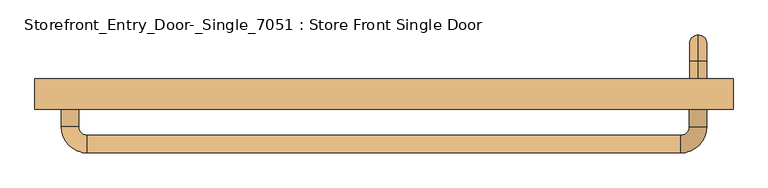
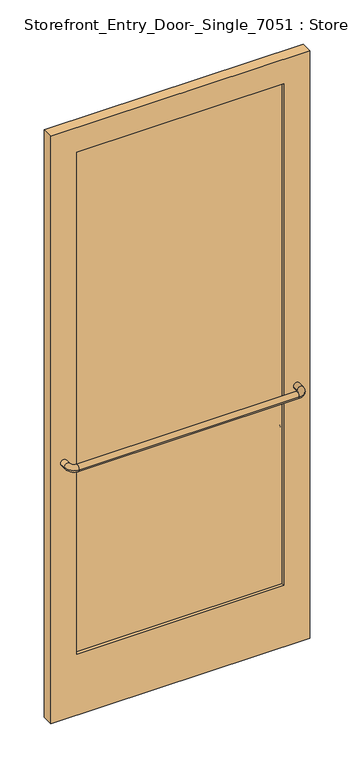
"""IFC4 building model written with IfcOpenShell, lengths in millimetres: door geometry, Storefront_Entry_Door-_Single_7051 : Store Front Single Door."""

from ifc_helpers import new_model, si_unit, point, frame, origin, place, context, project, spatial, polyline, circle_curve, ellipse_curve, trimmed, outline, extrude, source, transform, mapped, element, save
from ifc_brep_helpers import plane_surface, cylinder_surface, revolved_surface, advanced_brep


def storefront_entry_door_single_7051_store_front_single_door_f67f6f5c(model_context):
    return source(origin(), model_context, "Body", "SolidModel", [
        advanced_brep(
        [(457.2, 50.8, 1054.1), (457.2, 50.8, 1079.5), (457.2, 76.2, 1054.1), (457.2, 76.2, 1079.5), (457.2, 114.3, 1041.4), (457.2, 88.9, 1041.4), (457.2, 88.9, 863.6), (457.2, 114.3, 863.6), (457.2, 76.2, 825.5), (457.2, 76.2, 850.9), (457.2, 50.8, 850.9), (457.2, 50.8, 825.5)],
        [
            (0, 1, circle_curve(frame((457.2, 50.8, 1066.8), z_axis=(0.0, -1.0, 0.0), x_axis=(0.0, 0.0, 1.0)), 12.7)),
            (1, 0, circle_curve(frame((457.2, 50.8, 1066.8), z_axis=(0.0, -1.0, 0.0), x_axis=(0.0, 0.0, 1.0)), 12.7)),
            (0, 2),
            (2, 3, circle_curve(frame((457.2, 76.2, 1066.8), z_axis=(0.0, -1.0, 0.0), x_axis=(0.0, 0.0, 1.0)), 12.7)),
            (3, 1),
            (3, 2, circle_curve(frame((457.2, 76.2, 1066.8), z_axis=(0.0, -1.0, 0.0), x_axis=(0.0, 0.0, 1.0)), 12.7)),
            (4, 3, circle_curve(frame((457.2, 76.2, 1041.4), z_axis=(1.0, 0.0, 0.0), x_axis=(0.0, 0.0, 1.0)), 38.1)),
            (2, 5, circle_curve(frame((457.2, 76.2, 1041.4), z_axis=(-1.0, 0.0, 0.0), x_axis=(0.0, 0.0, 1.0)), 12.7)),
            (5, 4, circle_curve(frame((457.2, 101.6, 1041.4), z_axis=(0.0, 0.0, 1.0), x_axis=(0.0, 1.0, 0.0)), 12.7)),
            (4, 5, circle_curve(frame((457.2, 101.6, 1041.4), z_axis=(0.0, 0.0, 1.0), x_axis=(0.0, 1.0, 0.0)), 12.7)),
            (5, 6),
            (6, 7, circle_curve(frame((457.2, 101.6, 863.6), z_axis=(0.0, 0.0, 1.0), x_axis=(0.0, 1.0, 0.0)), 12.7)),
            (7, 4),
            (7, 6, circle_curve(frame((457.2, 101.6, 863.6), z_axis=(0.0, 0.0, 1.0), x_axis=(0.0, 1.0, 0.0)), 12.7)),
            (8, 7, circle_curve(frame((457.2, 76.2, 863.6), z_axis=(1.0, 0.0, 0.0), x_axis=(0.0, 1.0, 0.0)), 38.1)),
            (6, 9, circle_curve(frame((457.2, 76.2, 863.6), z_axis=(-1.0, 0.0, 0.0), x_axis=(0.0, 1.0, 0.0)), 12.7)),
            (9, 8, circle_curve(frame((457.2, 76.2, 838.2), z_axis=(0.0, 1.0, 0.0), x_axis=(0.0, 0.0, -1.0)), 12.7)),
            (8, 9, circle_curve(frame((457.2, 76.2, 838.2), z_axis=(0.0, 1.0, 0.0), x_axis=(0.0, 0.0, -1.0)), 12.7)),
            (10, 11, circle_curve(frame((457.2, 50.8, 838.2), z_axis=(0.0, -1.0, 0.0), x_axis=(0.0, 0.0, -1.0)), 12.7)),
            (11, 10, circle_curve(frame((457.2, 50.8, 838.2), z_axis=(0.0, -1.0, 0.0), x_axis=(0.0, 0.0, -1.0)), 12.7)),
            (9, 10),
            (11, 8),
        ],
        [
            plane_surface(frame((457.2, 50.8, 1066.8), z_axis=(0.0, -1.0, 0.0), x_axis=(1.0, 0.0, 0.0))),
            cylinder_surface(frame((457.2, 50.8, 1066.8), z_axis=(0.0, -1.0, 0.0), x_axis=(0.0, 0.0, 1.0)), 12.7),
            revolved_surface(trimmed(ellipse_curve(frame((457.2, 76.2, 1066.8), z_axis=(0.0, -1.0, 0.0), x_axis=(0.0, 0.0, 1.0)), 12.7, 12.7), [point((457.2, 76.2, 1054.1))], [point((457.2, 76.2, 1079.5))], True, "CARTESIAN"), (457.2, 76.2, 1041.4), (-1.0, 0.0, 0.0)),
            revolved_surface(trimmed(ellipse_curve(frame((457.2, 76.2, 1066.8), z_axis=(0.0, -1.0, 0.0), x_axis=(0.0, 0.0, 1.0)), 12.7, 12.7), [point((457.2, 76.2, 1079.5))], [point((457.2, 76.2, 1054.1))], True, "CARTESIAN"), (457.2, 76.2, 1041.4), (-1.0, 0.0, 0.0)),
            cylinder_surface(frame((457.2, 101.6, 1041.4), z_axis=(0.0, 0.0, 1.0), x_axis=(0.0, 1.0, 0.0)), 12.7),
            revolved_surface(trimmed(ellipse_curve(frame((457.2, 101.6, 863.6), z_axis=(0.0, 0.0, 1.0), x_axis=(0.0, 1.0, 0.0)), 12.7, 12.7), [point((457.2, 88.9, 863.6))], [point((457.2, 114.3, 863.6))], True, "CARTESIAN"), (457.2, 76.2, 863.6), (-1.0, 0.0, 0.0)),
            revolved_surface(trimmed(ellipse_curve(frame((457.2, 101.6, 863.6), z_axis=(0.0, 0.0, 1.0), x_axis=(0.0, 1.0, 0.0)), 12.7, 12.7), [point((457.2, 114.3, 863.6))], [point((457.2, 88.9, 863.6))], True, "CARTESIAN"), (457.2, 76.2, 863.6), (-1.0, 0.0, 0.0)),
            plane_surface(frame((457.2, 50.8, 838.2), z_axis=(0.0, -1.0, 0.0), x_axis=(1.0, 0.0, 0.0))),
            cylinder_surface(frame((457.2, 76.2, 838.2), z_axis=(0.0, 1.0, 0.0), x_axis=(0.0, 0.0, -1.0)), 12.7),
        ],
        [
            (0, [[1, 2]]),
            (1, [[-1, 3, 4, 5]]),
            (1, [[-2, -5, 6, -3]]),
            (2, [[7, -4, 8, 9]]),
            (3, [[-8, -6, -7, 10]]),
            (4, [[-9, 11, 12, 13]]),
            (4, [[-10, -13, 14, -11]]),
            (5, [[15, -12, 16, 17]]),
            (6, [[-16, -14, -15, 18]]),
            (7, [[19, 20]]),
            (8, [[-17, 21, -20, 22]]),
            (8, [[-18, -22, -19, -21]]),
        ],
    ),
        advanced_brep(
        [(444.5, 6.35, 1066.8), (469.9, 6.35, 1066.8), (444.5, -19.05, 1066.8), (469.9, -19.05, 1066.8), (431.8, -57.15, 1066.8), (431.8, -31.75, 1066.8), (-431.8, -31.75, 1066.8), (-431.8, -57.15, 1066.8), (-469.9, -19.05, 1066.8), (-444.5, -19.05, 1066.8), (-444.5, 6.35, 1066.8), (-469.9, 6.35, 1066.8)],
        [
            (0, 1, circle_curve(frame((457.2, 6.35, 1066.8), z_axis=(0.0, 1.0, 0.0), x_axis=(1.0, 0.0, 0.0)), 12.7)),
            (1, 0, circle_curve(frame((457.2, 6.35, 1066.8), z_axis=(0.0, 1.0, 0.0), x_axis=(1.0, 0.0, 0.0)), 12.7)),
            (0, 2),
            (2, 3, circle_curve(frame((457.2, -19.05, 1066.8), z_axis=(0.0, 1.0, 0.0), x_axis=(1.0, 0.0, 0.0)), 12.7)),
            (3, 1),
            (3, 2, circle_curve(frame((457.2, -19.05, 1066.8), z_axis=(0.0, 1.0, 0.0), x_axis=(1.0, 0.0, 0.0)), 12.7)),
            (4, 3, circle_curve(frame((431.8, -19.05, 1066.8), z_axis=(0.0, 0.0, 1.0), x_axis=(1.0, 0.0, 0.0)), 38.1)),
            (2, 5, circle_curve(frame((431.8, -19.05, 1066.8), z_axis=(0.0, 0.0, -1.0), x_axis=(1.0, 0.0, 0.0)), 12.7)),
            (5, 4, circle_curve(frame((431.8, -44.45, 1066.8), z_axis=(1.0, 0.0, 0.0), x_axis=(0.0, -1.0, 0.0)), 12.7)),
            (4, 5, circle_curve(frame((431.8, -44.45, 1066.8), z_axis=(1.0, 0.0, 0.0), x_axis=(0.0, -1.0, 0.0)), 12.7)),
            (5, 6),
            (6, 7, circle_curve(frame((-431.8, -44.45, 1066.8), z_axis=(1.0, 0.0, 0.0), x_axis=(0.0, -1.0, 0.0)), 12.7)),
            (7, 4),
            (7, 6, circle_curve(frame((-431.8, -44.45, 1066.8), z_axis=(1.0, 0.0, 0.0), x_axis=(0.0, -1.0, 0.0)), 12.7)),
            (8, 7, circle_curve(frame((-431.8, -19.05, 1066.8), z_axis=(0.0, 0.0, 1.0), x_axis=(0.0, -1.0, 0.0)), 38.1)),
            (6, 9, circle_curve(frame((-431.8, -19.05, 1066.8), z_axis=(0.0, 0.0, -1.0), x_axis=(0.0, -1.0, 0.0)), 12.7)),
            (9, 8, circle_curve(frame((-457.2, -19.05, 1066.8), z_axis=(0.0, -1.0, 0.0), x_axis=(-1.0, 0.0, 0.0)), 12.7)),
            (8, 9, circle_curve(frame((-457.2, -19.05, 1066.8), z_axis=(0.0, -1.0, 0.0), x_axis=(-1.0, 0.0, 0.0)), 12.7)),
            (10, 11, circle_curve(frame((-457.2, 6.35, 1066.8), z_axis=(0.0, 1.0, 0.0), x_axis=(-1.0, 0.0, 0.0)), 12.7)),
            (11, 10, circle_curve(frame((-457.2, 6.35, 1066.8), z_axis=(0.0, 1.0, 0.0), x_axis=(-1.0, 0.0, 0.0)), 12.7)),
            (9, 10),
            (11, 8),
        ],
        [
            plane_surface(frame((457.2, 6.35, 1066.8), z_axis=(0.0, 1.0, 0.0), x_axis=(0.0, 0.0, 1.0))),
            cylinder_surface(frame((457.2, 6.35, 1066.8), z_axis=(0.0, 1.0, 0.0), x_axis=(1.0, 0.0, 0.0)), 12.7),
            revolved_surface(trimmed(ellipse_curve(frame((457.2, -19.05, 1066.8), z_axis=(0.0, 1.0, 0.0), x_axis=(1.0, 0.0, 0.0)), 12.7, 12.7), [point((444.5, -19.05, 1066.8))], [point((469.9, -19.05, 1066.8))], True, "CARTESIAN"), (431.8, -19.05, 1066.8), (0.0, 0.0, -1.0)),
            revolved_surface(trimmed(ellipse_curve(frame((457.2, -19.05, 1066.8), z_axis=(0.0, 1.0, 0.0), x_axis=(1.0, 0.0, 0.0)), 12.7, 12.7), [point((469.9, -19.05, 1066.8))], [point((444.5, -19.05, 1066.8))], True, "CARTESIAN"), (431.8, -19.05, 1066.8), (0.0, 0.0, -1.0)),
            cylinder_surface(frame((431.8, -44.45, 1066.8), z_axis=(1.0, 0.0, 0.0), x_axis=(0.0, -1.0, 0.0)), 12.7),
            revolved_surface(trimmed(ellipse_curve(frame((-431.8, -44.45, 1066.8), z_axis=(1.0, 0.0, 0.0), x_axis=(0.0, -1.0, 0.0)), 12.7, 12.7), [point((-431.8, -31.75, 1066.8))], [point((-431.8, -57.15, 1066.8))], True, "CARTESIAN"), (-431.8, -19.05, 1066.8), (0.0, 0.0, -1.0)),
            revolved_surface(trimmed(ellipse_curve(frame((-431.8, -44.45, 1066.8), z_axis=(1.0, 0.0, 0.0), x_axis=(0.0, -1.0, 0.0)), 12.7, 12.7), [point((-431.8, -57.15, 1066.8))], [point((-431.8, -31.75, 1066.8))], True, "CARTESIAN"), (-431.8, -19.05, 1066.8), (0.0, 0.0, -1.0)),
            plane_surface(frame((-457.2, 6.35, 1066.8), z_axis=(0.0, 1.0, 0.0), x_axis=(0.0, 0.0, 1.0))),
            cylinder_surface(frame((-457.2, -19.05, 1066.8), z_axis=(0.0, -1.0, 0.0), x_axis=(-1.0, 0.0, 0.0)), 12.7),
        ],
        [
            (0, [[1, 2]]),
            (1, [[-1, 3, 4, 5]]),
            (1, [[-2, -5, 6, -3]]),
            (2, [[7, -4, 8, 9]]),
            (3, [[-8, -6, -7, 10]]),
            (4, [[-9, 11, 12, 13]]),
            (4, [[-10, -13, 14, -11]]),
            (5, [[15, -12, 16, 17]]),
            (6, [[-16, -14, -15, 18]]),
            (7, [[19, 20]]),
            (8, [[-17, 21, -20, 22]]),
            (8, [[-18, -22, -19, -21]]),
        ],
    ),
        extrude(outline(polyline([(406.4, 19.05), (-406.4, 19.05), (-406.4, 38.1), (406.4, 38.1), (406.4, 19.05)])), frame((0.0, 0.0, 254.0), z_axis=(0.0, 0.0, 1.0), x_axis=(1.0, 0.0, 0.0)), (0.0, 0.0, 1.0), 2082.8),
        extrude(outline(polyline([(2438.4, 508.0), (2438.4, -508.0), (0.0, -508.0), (0.0, 508.0), (2438.4, 508.0)]), holes=[polyline([(2336.8, -406.4), (2336.8, 406.4), (254.0, 406.4), (254.0, -406.4), (2336.8, -406.4)])]), frame((0.0, 6.35, 0.0), z_axis=(0.0, 1.0, 0.0), x_axis=(0.0, 0.0, 1.0)), (0.0, 0.0, 1.0), 44.45),
    ])


if __name__ == "__main__":
    model = new_model("IFC4")
    model_context = context("Model", 3, world=origin())
    ifc_project = project(units=[si_unit("LENGTHUNIT", "METRE", prefix="MILLI")], contexts=[model_context])
    site = spatial("IfcSite", under=ifc_project)
    building = spatial("IfcBuilding", under=site)
    placement = place(None, origin())
    storefront_entry_door_single_7051_store_front_single_door_shape = storefront_entry_door_single_7051_store_front_single_door_f67f6f5c(model_context)
    element("IfcDoor", 1, ObjectType="Storefront_Entry_Door-_Single_7051 : Store Front Single Door", at=placement, inside=building, context=model_context, shape_type="MappedRepresentation", body=[
        mapped(storefront_entry_door_single_7051_store_front_single_door_shape, transform((0.0, 0.0, 0.0), x_axis=(1.0, 0.0, 0.0), y_axis=(0.0, 1.0, 0.0), z_axis=(0.0, 0.0, 1.0))),
    ])
    save(model, "model.ifc")

# Revit data of these elements
# Type "Storefront_Entry_Door-_Single_7051 : Store Front Single Door"
#   Type Comments = "TEMPERED GLAZING"
#   Type Mark = "19"
#   Assembly Code = "B2030110"
#   Analytic Construction = "<None>"
#   Top Rail = 0' - 4"
#   Side Rail = 0' - 4"
#   Reporting Width [instance default] = 4' - 2"
#   Rail Height AFF = 3' - 6"
#   Offset = 0' - 2"
#   Door Width [instance default] = 4' - 2"
#   Bottom Rail Width = 0' - 10"
#   Material = Metal - Aluminum
#   Glazing Material = Glass
#   Function = (empty or 0)
# Element 1 (IfcDoor, "Storefront_Entry_Door-_Single_7051 : Store Front Single Door")
#   Reporting Width = 3' - 4"
#   Door Width = 3' - 4"
#   Materials on its faces: "Metal - Aluminum", "Glass"
# Materials
#   "Metal - Aluminum": class "Metal", colour RGB 247 247 247, transparency 0
#   "Glass": class "Glass", colour RGB 218 227 224, transparency 0.85, Description = "Soda Lime Glass", Cost = 0
